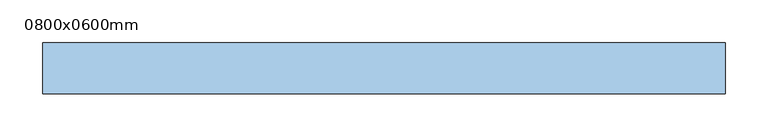
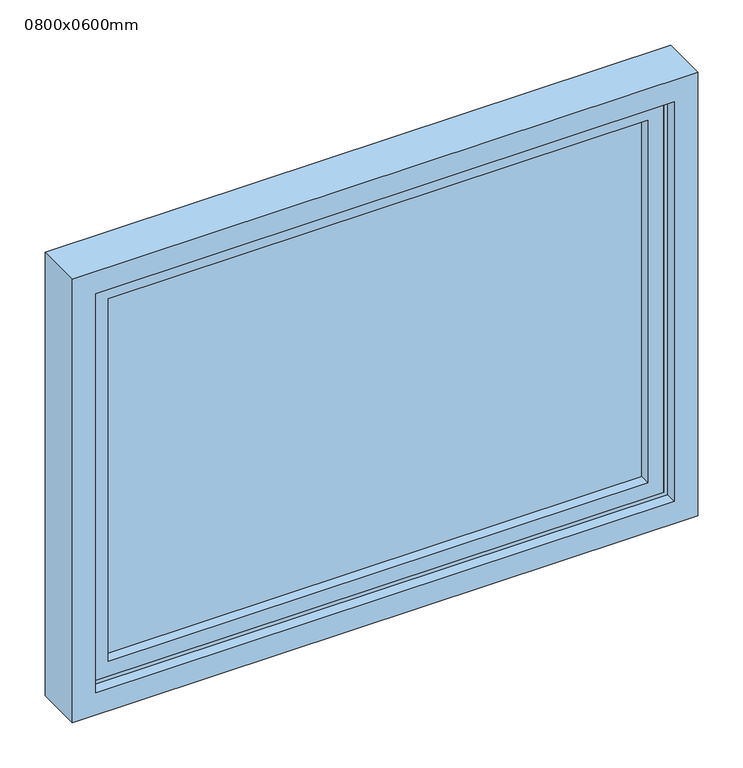
"""IFC4 building model written with IfcOpenShell, lengths in millimetres: window geometry, Janela Maxim-air - 1 Módulo : 0800x0600mm."""

import ifcopenshell
import ifcopenshell.guid

model = None  # the IFC model being written
_history = None  # IfcOwnerHistory: only IFC2X3 demands one
_inside = {}  # id of a spatial element -> (the spatial element, [elements in it])
_under = {}  # id of a project, library or spatial element -> (it, [spatial elements below it])
_declared = {}  # id of a project -> (the project, [libraries it declares])
_typed = {}  # id of a type object -> (the type object, [elements of that type])
_made_of = {}  # id of a material, layer set ... -> (it, [elements and type objects made of it])


def new_model(schema):
    """Start an empty IFC model of exactly this schema.

    Asked for "IFC4X3", IfcOpenShell would pick the latest addendum, in which some entities
    have other attributes; the version numbers below select the first issue.
    IFC2X3 requires an IfcOwnerHistory on every rooted entity: one is made here for all.
    """
    global model, _history
    if schema == "IFC4X3":
        model = ifcopenshell.file(schema_version=(4, 3, 0, 0))
    else:
        model = ifcopenshell.file(schema=schema)
    _inside.clear()
    _under.clear()
    _declared.clear()
    _typed.clear()
    _made_of.clear()
    _history = None
    if model.schema == "IFC2X3":
        org = make("IfcOrganization", Name="unknown")
        user = make(
            "IfcPersonAndOrganization",
            ThePerson=make("IfcPerson", FamilyName="unknown"),
            TheOrganization=org,
        )
        app = make(
            "IfcApplication",
            ApplicationDeveloper=org,
            Version="unknown",
            ApplicationFullName="unknown",
            ApplicationIdentifier="unknown",
        )
        _history = make(
            "IfcOwnerHistory",
            OwningUser=user,
            OwningApplication=app,
            ChangeAction="ADDED",
            CreationDate=0,
        )
    return model


def make(cls, **values):
    """One entity of the class cls with the attributes given. An attribute that is None is left unset."""
    return model.create_entity(
        cls, **{name: value for name, value in values.items() if value is not None}
    )


def rooted(cls, **values):
    """An entity with a GlobalId (a new one), such as an element, a storey or a relation."""
    return make(cls, GlobalId=ifcopenshell.guid.new(), OwnerHistory=_history, **values)


def si_unit(unit_type, name, prefix=None):
    """IfcSIUnit, for example si_unit("LENGTHUNIT", "METRE", prefix="MILLI")."""
    return make("IfcSIUnit", UnitType=unit_type, Prefix=prefix, Name=name)


def assignment(units):
    """IfcUnitAssignment: the units of a project."""
    return None if units is None else make("IfcUnitAssignment", Units=units)


def point(xyz):
    """IfcCartesianPoint."""
    return None if xyz is None else make("IfcCartesianPoint", Coordinates=xyz)


def direction(xyz):
    """IfcDirection."""
    return None if xyz is None else make("IfcDirection", DirectionRatios=xyz)


def frame(location, z_axis=None, x_axis=None):
    """IfcAxis2Placement3D, a coordinate frame: its origin and axes. An axis left out is left unset."""
    return make(
        "IfcAxis2Placement3D",
        Location=point(location),
        Axis=direction(z_axis),
        RefDirection=direction(x_axis),
    )


def origin():
    """The frame at (0, 0, 0) with its axes left unset."""
    return frame((0.0, 0.0, 0.0))


def place(relative_to, where):
    """IfcLocalPlacement: puts the frame where relative to a parent placement (None: the world)."""
    return make(
        "IfcLocalPlacement", PlacementRelTo=relative_to, RelativePlacement=where
    )


def context(
    kind, dimensions, precision=None, world=None, true_north=None, identifier=None
):
    """IfcGeometricRepresentationContext, for example the 3D "Model" context."""
    return make(
        "IfcGeometricRepresentationContext",
        ContextIdentifier=identifier,
        ContextType=kind,
        CoordinateSpaceDimension=dimensions,
        Precision=precision,
        WorldCoordinateSystem=world,
        TrueNorth=true_north,
    )


def project(units=None, contexts=None):
    """IfcProject with its units and contexts."""
    return rooted(
        "IfcProject",
        Name="project",
        RepresentationContexts=contexts,
        UnitsInContext=assignment(units),
    )


def spatial(cls, under=None, at=None, **own):
    """A site, building, storey or space (cls), placed at a placement, below another one or the project."""
    s = rooted(cls, ObjectPlacement=at, **own)
    if under is not None:
        _under.setdefault(under.id(), (under, []))[1].append(s)
    return s


def polyline(points):
    """IfcPolyline through the points."""
    return make("IfcPolyline", Points=[point(p) for p in points])


def outline(outer, holes=None, kind="AREA"):
    """IfcArbitraryClosedProfileDef: a profile drawn as a closed curve; with holes, ...WithVoids."""
    if holes is None:
        return make("IfcArbitraryClosedProfileDef", ProfileType=kind, OuterCurve=outer)
    return make(
        "IfcArbitraryProfileDefWithVoids",
        ProfileType=kind,
        OuterCurve=outer,
        InnerCurves=holes,
    )


def extrude(swept, where, along, depth):
    """IfcExtrudedAreaSolid: the profile swept, set in the frame where, extruded along a direction by depth."""
    return make(
        "IfcExtrudedAreaSolid",
        SweptArea=swept,
        Position=where,
        ExtrudedDirection=direction(along),
        Depth=depth,
    )


def faces_of(points, faces, orient=None, outer=None):
    """IfcFace entities. A face is a list of loops; a loop is a list of indices into points, from 0.

    orient and outer hold one flag for each loop. By default every Orientation is true, the
    first loop of a face is its IfcFaceOuterBound and the others are IfcFaceBound.
    """
    made = []
    for i, loops in enumerate(faces):
        bounds = []
        for j, loop in enumerate(loops):
            is_outer = j == 0 if outer is None else outer[i][j]
            bounds.append(
                make(
                    "IfcFaceOuterBound" if is_outer else "IfcFaceBound",
                    Bound=make("IfcPolyLoop", Polygon=[points[k] for k in loop]),
                    Orientation=True if orient is None else orient[i][j],
                )
            )
        made.append(make("IfcFace", Bounds=bounds))
    return made


def faceted_brep(points, faces, orient=None, outer=None, voids=None):
    """IfcFacetedBrep: a solid bounded by flat faces; with voids (closed shells), ...WithVoids."""
    shared = [point(p) for p in points]
    hull = make("IfcClosedShell", CfsFaces=faces_of(shared, faces, orient, outer))
    if voids is None:
        return make("IfcFacetedBrep", Outer=hull)
    return make(
        "IfcFacetedBrepWithVoids",
        Outer=hull,
        Voids=[
            make(cls, CfsFaces=faces_of(shared, fs, o, b)) for cls, fs, o, b in voids
        ],
    )


def shape(context_of_items, identifier, shape_type, items):
    """IfcShapeRepresentation: the items that make up one representation, for example the "Body"."""
    return make(
        "IfcShapeRepresentation",
        ContextOfItems=context_of_items,
        RepresentationIdentifier=identifier,
        RepresentationType=shape_type,
        Items=items,
    )


def source(mapping_origin, context_of_items, identifier, shape_type, items):
    """IfcRepresentationMap: a shape defined once, which mapped items show again and again."""
    return make(
        "IfcRepresentationMap",
        MappingOrigin=mapping_origin,
        MappedRepresentation=shape(context_of_items, identifier, shape_type, items),
    )


def transform(
    local_origin,
    x_axis=None,
    y_axis=None,
    z_axis=None,
    scale=None,
    scale2=None,
    scale3=None,
    uniform=True,
):
    """IfcCartesianTransformationOperator3D, or its non-uniform kind. x_axis, y_axis, z_axis: its Axis1, 2, 3."""
    if uniform:
        return make(
            "IfcCartesianTransformationOperator3D",
            Axis1=direction(x_axis),
            Axis2=direction(y_axis),
            LocalOrigin=point(local_origin),
            Scale=scale,
            Axis3=direction(z_axis),
        )
    return make(
        "IfcCartesianTransformationOperator3DnonUniform",
        Axis1=direction(x_axis),
        Axis2=direction(y_axis),
        LocalOrigin=point(local_origin),
        Scale=scale,
        Axis3=direction(z_axis),
        Scale2=scale2,
        Scale3=scale3,
    )


def mapped(mapping_source, mapping_target):
    """IfcMappedItem: shows the shape of a source again, moved by a transform."""
    return make(
        "IfcMappedItem", MappingSource=mapping_source, MappingTarget=mapping_target
    )


def made_of(thing, what):
    """Note that an element or type object is made of a material, layer set ...; save() writes the relation."""
    if what is not None:
        _made_of.setdefault(what.id(), (what, []))[1].append(thing)
    return thing


def element(
    cls,
    number,
    at=None,
    inside=None,
    cuts=None,
    type_object=None,
    material=None,
    context=None,
    identifier="Body",
    shape_type=None,
    held_by="IfcProductDefinitionShape",
    body=None,
    shapes=None,
    **own,
):
    """One element of the class cls, such as IfcWall. Its Tag is "e" and its number.

    at: its placement. inside: the storey or other place that contains it. cuts: it is an
    opening in that element (IfcRelVoidsElement). A single representation is given by context,
    identifier, shape_type and body (its items); several are given by shapes. held_by: the class
    of the entity that holds the representations. save() writes the other relations.
    """
    e = rooted(cls, Tag="e%d" % number, ObjectPlacement=at, **own)
    if body is not None:
        shapes = [shape(context, identifier, shape_type, body)]
    if shapes is not None:
        e.Representation = make(held_by, Representations=shapes)
    if inside is not None:
        _inside.setdefault(inside.id(), (inside, []))[1].append(e)
    if cuts is not None:
        rooted(
            "IfcRelVoidsElement", RelatingBuildingElement=cuts, RelatedOpeningElement=e
        )
    if type_object is not None:
        _typed.setdefault(type_object.id(), (type_object, []))[1].append(e)
    return made_of(e, material)


def aggregate(whole, parts):
    """IfcRelAggregates: a whole, such as a stair, and the parts it consists of."""
    return rooted("IfcRelAggregates", RelatingObject=whole, RelatedObjects=parts)


def save(model, path):
    """Write the relations noted so far, then the file.

    IfcRelAggregates (storeys below a building ...), IfcRelContainedInSpatialStructure (elements
    in a storey), IfcRelDefinesByType, IfcRelAssociatesMaterial and IfcRelDeclares: one each for
    every whole, place, type object, material and project.
    """
    for whole, parts in _under.values():
        aggregate(whole, parts)
    for where, things in _inside.values():
        rooted(
            "IfcRelContainedInSpatialStructure",
            RelatedElements=things,
            RelatingStructure=where,
        )
    for kind, things in _typed.values():
        rooted("IfcRelDefinesByType", RelatedObjects=things, RelatingType=kind)
    for what, things in _made_of.values():
        rooted("IfcRelAssociatesMaterial", RelatedObjects=things, RelatingMaterial=what)
    for by, libraries in _declared.values():
        rooted("IfcRelDeclares", RelatingContext=by, RelatedDefinitions=libraries)
    model.write(path)


def window_0800x0600mm_eab3bed5(model_context):
    return source(origin(), model_context, "Body", "SolidModel", [
        extrude(outline(polyline([(-352.0, -24.120858), (352.0, -24.120858), (352.0, -31.120858), (-352.0, -31.120858), (-352.0, -24.120858)])), frame((0.0, 0.0, 1048.0), z_axis=(0.0, 0.0, 1.0), x_axis=(1.0, 0.0, 0.0)), (0.0, 0.0, 1.0), 504.0),
        faceted_brep([(345.0, -45.120858, 1545.0), (345.0, -31.120858, 1545.0), (345.0, -31.120858, 1055.0), (345.0, -45.120858, 1055.0), (352.0, -31.120858, 1552.0), (352.0, -24.120858, 1552.0), (352.0, -24.120858, 1048.0), (352.0, -31.120858, 1048.0), (345.0, -24.120858, 1545.0), (345.0, -10.120858, 1545.0), (345.0, -10.120858, 1055.0), (345.0, -24.120858, 1055.0), (365.0, -10.120858, 1565.0), (365.0, -45.120858, 1565.0), (365.0, -45.120858, 1035.0), (365.0, -10.120858, 1035.0), (-345.0, -31.120858, 1055.0), (-345.0, -45.120858, 1055.0), (-352.0, -24.120858, 1048.0), (-352.0, -31.120858, 1048.0), (-345.0, -10.120858, 1055.0), (-345.0, -24.120858, 1055.0), (-365.0, -45.120858, 1035.0), (-365.0, -10.120858, 1035.0), (-345.0, -31.120858, 1545.0), (-345.0, -45.120858, 1545.0), (-352.0, -24.120858, 1552.0), (-352.0, -31.120858, 1552.0), (-345.0, -10.120858, 1545.0), (-345.0, -24.120858, 1545.0), (-365.0, -45.120858, 1565.0), (-365.0, -10.120858, 1565.0)], [[[0, 1, 2, 3]], [[4, 5, 6, 7]], [[8, 9, 10, 11]], [[12, 13, 14, 15]], [[3, 2, 16, 17]], [[7, 6, 18, 19]], [[11, 10, 20, 21]], [[15, 14, 22, 23]], [[17, 16, 24, 25]], [[19, 18, 26, 27]], [[21, 20, 28, 29]], [[23, 22, 30, 31]], [[13, 30, 22, 14], [3, 17, 25, 0]], [[25, 24, 1, 0]], [[7, 19, 27, 4], [1, 24, 16, 2]], [[27, 26, 5, 4]], [[5, 26, 18, 6], [11, 21, 29, 8]], [[29, 28, 9, 8]], [[15, 23, 31, 12], [9, 28, 20, 10]], [[31, 30, 13, 12]]]),
        faceted_brep([(365.0, -45.120858, 1565.0), (365.0, -10.120858, 1565.0), (365.0, -10.120858, 1035.0), (365.0, -45.120858, 1035.0), (360.0, -10.120858, 1560.0), (360.0, -5.120858, 1560.0), (360.0, -5.120858, 1040.0), (360.0, -10.120858, 1040.0), (370.0, -5.120858, 1570.0), (370.0, -45.120858, 1570.0), (370.0, -45.120858, 1030.0), (370.0, -5.120858, 1030.0), (-365.0, -10.120858, 1035.0), (-365.0, -45.120858, 1035.0), (-360.0, -5.120858, 1040.0), (-360.0, -10.120858, 1040.0), (-370.0, -45.120858, 1030.0), (-370.0, -5.120858, 1030.0), (-365.0, -10.120858, 1565.0), (-365.0, -45.120858, 1565.0), (-360.0, -5.120858, 1560.0), (-360.0, -10.120858, 1560.0), (-370.0, -45.120858, 1570.0), (-370.0, -5.120858, 1570.0)], [[[0, 1, 2, 3]], [[4, 5, 6, 7]], [[8, 9, 10, 11]], [[3, 2, 12, 13]], [[7, 6, 14, 15]], [[11, 10, 16, 17]], [[13, 12, 18, 19]], [[15, 14, 20, 21]], [[17, 16, 22, 23]], [[9, 22, 16, 10], [3, 13, 19, 0]], [[19, 18, 1, 0]], [[1, 18, 12, 2], [7, 15, 21, 4]], [[21, 20, 5, 4]], [[11, 17, 23, 8], [5, 20, 14, 6]], [[23, 22, 9, 8]]]),
        faceted_brep([(400.0, -0.120858, 1600.0), (400.0, -60.120858, 1600.0), (400.0, -60.120858, 1000.0), (400.0, -0.120858, 1000.0), (-400.0, -60.120858, 1600.0), (-400.0, -60.120858, 1000.0), (370.0, -60.120858, 1030.0), (-370.0, -60.120858, 1030.0), (-370.0, -60.120858, 1570.0), (370.0, -60.120858, 1570.0), (-400.0, -0.120858, 1000.0), (-400.0, -0.120858, 1600.0), (360.0, -0.120858, 1560.0), (-360.0, -0.120858, 1560.0), (-360.0, -0.120858, 1040.0), (360.0, -0.120858, 1040.0), (370.0, -5.120858, 1570.0), (370.0, -5.120858, 1030.0), (-370.0, -5.120858, 1570.0), (-370.0, -5.120858, 1030.0), (360.0, -5.120858, 1040.0), (-360.0, -5.120858, 1040.0), (-360.0, -5.120858, 1560.0), (360.0, -5.120858, 1560.0)], [[[0, 1, 2, 3]], [[1, 4, 5, 2], [6, 7, 8, 9]], [[3, 2, 5, 10]], [[3, 10, 11, 0], [12, 13, 14, 15]], [[9, 16, 17, 6]], [[16, 18, 19, 17], [20, 21, 22, 23]], [[6, 17, 19, 7]], [[10, 5, 4, 11]], [[7, 19, 18, 8]], [[23, 12, 15, 20]], [[20, 15, 14, 21]], [[21, 14, 13, 22]], [[11, 4, 1, 0]], [[8, 18, 16, 9]], [[22, 13, 12, 23]]]),
    ])


if __name__ == "__main__":
    model = new_model("IFC4")
    model_context = context("Model", 3, world=origin())
    ifc_project = project(units=[si_unit("LENGTHUNIT", "METRE", prefix="MILLI")], contexts=[model_context])
    site = spatial("IfcSite", under=ifc_project)
    building = spatial("IfcBuilding", under=site)
    placement = place(None, origin())
    window_0800x0600mm_shape = window_0800x0600mm_eab3bed5(model_context)
    element("IfcWindow", 1, ObjectType="Janela Maxim-air - 1 Módulo : 0800x0600mm", at=placement, inside=building, context=model_context, shape_type="MappedRepresentation", body=[
        mapped(window_0800x0600mm_shape, transform((0.0, 0.0, 0.0), x_axis=(1.0, 0.0, 0.0), y_axis=(0.0, 1.0, 0.0), z_axis=(0.0, 0.0, 1.0))),
    ])
    save(model, "model.ifc")

# Revit data of these elements
# Type "Janela Maxim-air - 1 Módulo : 0800x0600mm"
#   Type Mark = "19"
#   SINAPI = ""
#   Módulo Básico M = 0.10 m
#   Largura de Coordenação Modular CM = 0.80 m
#   Largura Painel = 0.74 m
#   Largura Batente = 0.06 m
#   Altura de Coordenação Modular CM = 0.60 m
#   Altura Peitoril = 1.00 m
#   Altura Painel = 0.54 m
#   Height = 0.60 m
#   Width = 0.80 m
#   Número de Módulos Básicos nM Largura = 8
#   Número de Módulos Básico nM Altura = 6
#   Material Quadro = Metal - Alumínio
#   Material Painel = Vidro
#   Wall Closure = (empty or 0)
#   Assembly Code = ""
# Element 1 (IfcWindow, "Janela Maxim-air - 1 Módulo : 0800x0600mm")
#   Materials on its faces: "Metal - Alumínio", "Vidro"
# Materials
#   "Metal - Alumínio": class "Metal", colour RGB 244 244 244, transparency 0
#   "Vidro": class "Vidro", colour RGB 0 128 192, transparency 0.9, Description = "Vidro de sílica", Cost = 0
